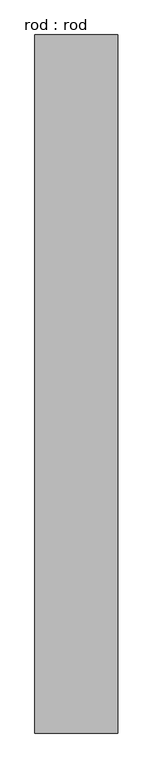
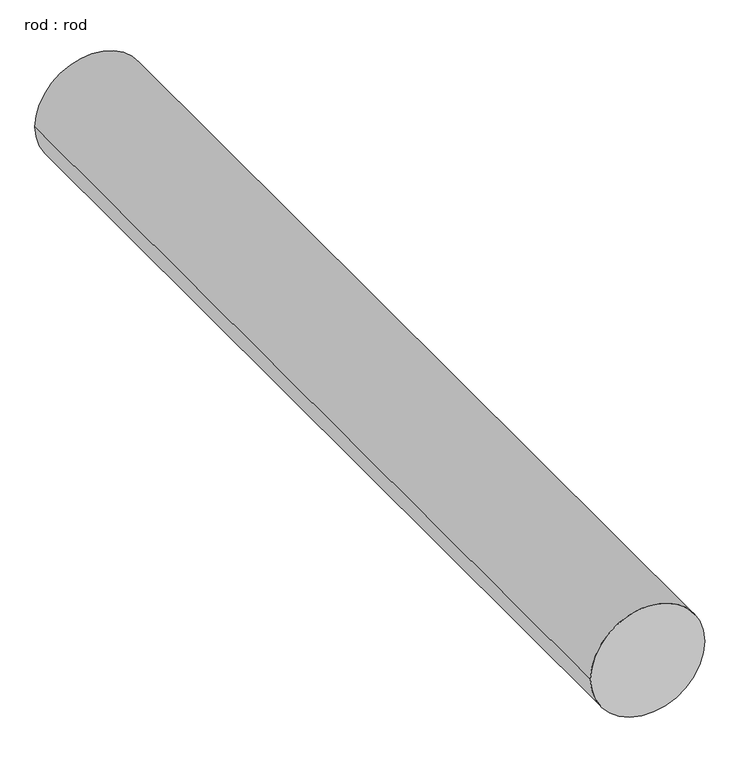
"""IFC4 building model written with IfcOpenShell, lengths in millimetres: proxy geometry, rod : rod."""

from ifc_helpers import new_model, si_unit, point, frame, frame_2d, origin, place, context, project, spatial, circle_curve, trimmed, segment, composite_curve, outline, extrude, source, transform, mapped, element, save


def rod_rod_40aea792(model_context):
    return source(origin(), model_context, "Body", "SweptSolid", [
        extrude(outline(composite_curve([segment(trimmed(circle_curve(frame_2d((0.0108462, 0.0)), 200.0), [point((0.0108462, 200.0))], [point((0.0108462, -200.0))], False, "CARTESIAN"), True, "CONTINUOUS"), segment(trimmed(circle_curve(frame_2d((0.0108462, 0.0)), 200.0), [point((0.0108462, -200.0))], [point((0.0108462, 200.0))], False, "CARTESIAN"), True, "CONTINUOUS")], self_intersect=False)), frame((0.0, 2405.2286153, 0.0), z_axis=(0.0, 1.0, 0.0), x_axis=(0.0, 0.0, 1.0)), (0.0, 0.0, 1.0), 3375.0),
    ])


if __name__ == "__main__":
    model = new_model("IFC4")
    model_context = context("Model", 3, world=origin())
    ifc_project = project(units=[si_unit("LENGTHUNIT", "METRE", prefix="MILLI")], contexts=[model_context])
    site = spatial("IfcSite", under=ifc_project)
    building = spatial("IfcBuilding", under=site)
    placement = place(None, origin())
    rod_rod_shape = rod_rod_40aea792(model_context)
    element("IfcBuildingElementProxy", 1, Name="rod : rod", ObjectType="rod : rod", at=placement, inside=building, context=model_context, shape_type="MappedRepresentation", body=[
        mapped(rod_rod_shape, transform((0.0, 0.0, 0.0), x_axis=(1.0, 0.0, 0.0), y_axis=(0.0, 1.0, 0.0), z_axis=(0.0, 0.0, 1.0))),
    ])
    save(model, "model.ifc")

# Revit data of these elements
# Type "rod : rod"
#   Default Elevation = 0
